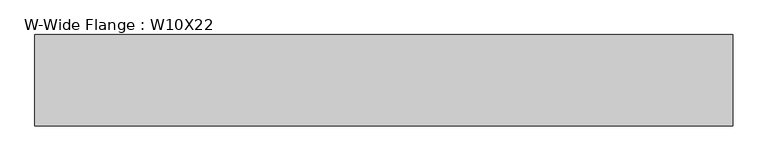
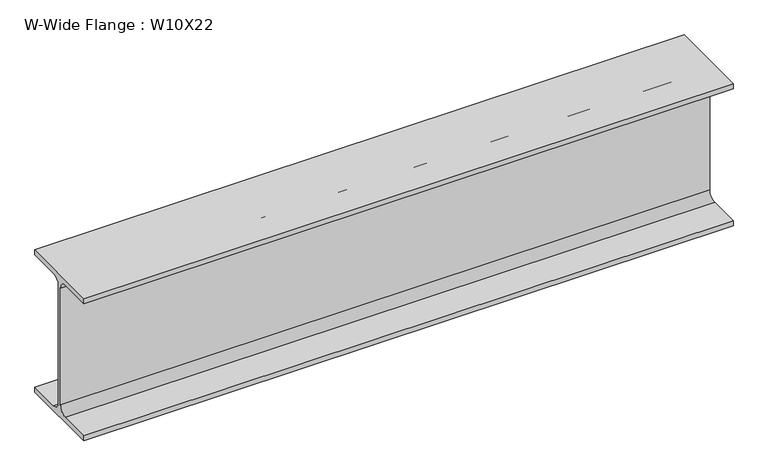
"""IFC4 building model written with IfcOpenShell, lengths in millimetres: beam geometry, W-Wide Flange : W10X22."""

from ifc_helpers import new_model, si_unit, point, frame, frame_2d, origin, place, context, project, spatial, polyline, circle_curve, trimmed, segment, composite_curve, outline, extrude, source, transform, mapped, element, save


def w_wide_flange_w10x22_c2580360(model_context):
    return source(origin(), model_context, "Body", "SweptSolid", [
        extrude(outline(composite_curve([segment(polyline([(73.025, -120.396), (73.025, -129.54), (-73.025, -129.54), (-73.025, -120.396), (-17.7165, -120.396)]), True, "CONTINUOUS"), segment(trimmed(circle_curve(frame_2d((-17.7165, -105.7275)), 14.6685), [point((-17.7165, -120.396))], [point((-3.048, -105.7275))], True, "CARTESIAN"), True, "CONTINUOUS"), segment(polyline([(-3.048, -105.7275), (-3.048, 105.7275)]), True, "CONTINUOUS"), segment(trimmed(circle_curve(frame_2d((-17.7165, 105.7275)), 14.6685), [point((-3.048, 105.7275))], [point((-17.7165, 120.396))], True, "CARTESIAN"), True, "CONTINUOUS"), segment(polyline([(-17.7165, 120.396), (-73.025, 120.396), (-73.025, 129.54), (73.025, 129.54), (73.025, 120.396), (17.7165, 120.396)]), True, "CONTINUOUS"), segment(trimmed(circle_curve(frame_2d((17.7165, 105.7275)), 14.6685), [point((17.7165, 120.396))], [point((3.048, 105.7275))], True, "CARTESIAN"), True, "CONTINUOUS"), segment(polyline([(3.048, 105.7275), (3.048, -105.7275)]), True, "CONTINUOUS"), segment(trimmed(circle_curve(frame_2d((17.7165, -105.7275)), 14.6685), [point((3.048, -105.7275))], [point((17.7165, -120.396))], True, "CARTESIAN"), True, "CONTINUOUS"), segment(polyline([(17.7165, -120.396), (73.025, -120.396)]), True, "CONTINUOUS")], self_intersect=False)), frame((-558.8, 0.0, 0.0), z_axis=(1.0, 0.0, 0.0), x_axis=(0.0, 1.0, 0.0)), (0.0, 0.0, 1.0), 1117.6),
    ])


if __name__ == "__main__":
    model = new_model("IFC4")
    model_context = context("Model", 3, world=origin())
    ifc_project = project(units=[si_unit("LENGTHUNIT", "METRE", prefix="MILLI")], contexts=[model_context])
    site = spatial("IfcSite", under=ifc_project)
    building = spatial("IfcBuilding", under=site)
    placement = place(None, origin())
    w_wide_flange_w10x22_shape = w_wide_flange_w10x22_c2580360(model_context)
    element("IfcBeam", 1, ObjectType="W-Wide Flange : W10X22", at=placement, inside=building, context=model_context, shape_type="MappedRepresentation", body=[
        mapped(w_wide_flange_w10x22_shape, transform((0.0, 0.0, 0.0), x_axis=(1.0, 0.0, 0.0), y_axis=(0.0, 1.0, 0.0), z_axis=(0.0, 0.0, 1.0))),
    ])
    save(model, "model.ifc")

# Revit data of these elements
# Type "W-Wide Flange : W10X22"
#   Assembly Code = "B10"
#   W = 22
#   Length [instance default] = 5' - 0"
#   bf = 0' - 5 3/4"
#   d = 0' - 10.2"
#   k = 0' - 0 15/16"
#   k2 = 0' - 0.5775"
#   tf = 0' - 0.36"
#   tw = 0' - 0.24"
#   A = 0.0450694 SF
#   Structural Material [instance default] = _STRUCTURAL STEEL (SEE STRUCT. DWGS)
# Element 1 (IfcBeam, "W-Wide Flange : W10X22")
#   Materials on its faces: "_STRUCTURAL STEEL (SEE STRUCT. DWGS)"
# Materials
#   "_STRUCTURAL STEEL (SEE STRUCT. DWGS)": class "Metal", colour RGB 199 199 199, transparency 0, Description = "Structural steel 50ksi", Cost = 0
